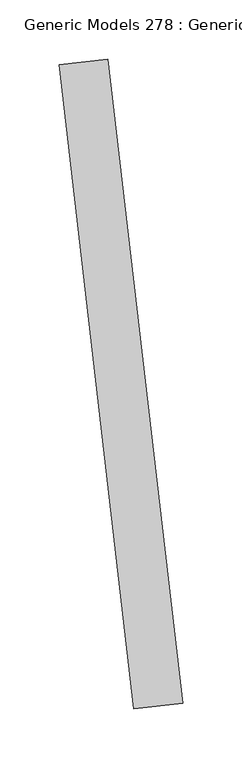
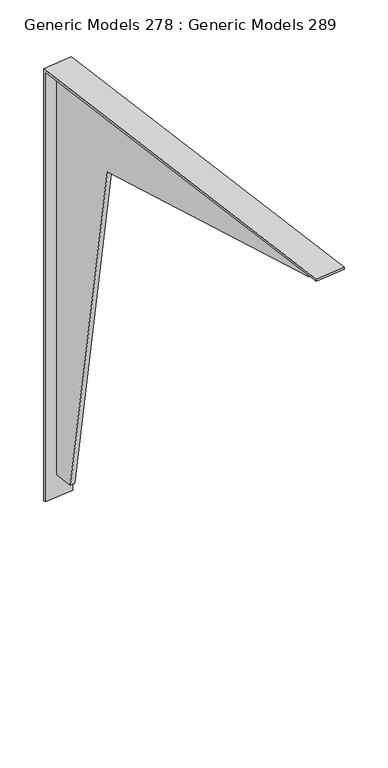
"""IFC4 building model written with IfcOpenShell, lengths in millimetres: proxy geometry, Generic Models 278 : Generic Models 289."""

from ifc_helpers import new_model, si_unit, frame, origin, place, context, project, spatial, polyline, outline, extrude, source, transform, mapped, element, save


def generic_models_278_generic_models_289_329f02fc(model_context):
    return source(origin(), model_context, "Body", "SweptSolid", [
        extrude(outline(polyline([(98.1060659, 0.0), (98.1060659, -596.4380662), (70.9315576, -596.4380662), (-3.4908021, -95.9091892), (-407.9025285, -22.6069609), (-407.9025285, 0.0), (98.1060659, 0.0)])), frame((-1150.4311232, -22429.6249942, 796.925), z_axis=(0.993316067089831, 0.11542612729009999, 0.0), x_axis=(-0.11542612729009999, 0.993316067089831, 0.0)), (0.0, 0.0, 1.0), 6.3961553),
        extrude(outline(polyline([(0.0, 0.0), (0.0, -547.7405886), (-632.0051767, -547.7405886), (-632.0051767, -544.6409847), (-3.175, -544.6409847), (-3.175, 0.0), (0.0, 0.0)])), frame((-1116.0829847, -22875.1732552, 800.1), z_axis=(0.993316067089831, 0.11542612729009999, 0.0), x_axis=(0.0, 0.0, 1.0)), (0.0, 0.0, 1.0), 41.275),
    ])


if __name__ == "__main__":
    model = new_model("IFC4")
    model_context = context("Model", 3, world=origin())
    ifc_project = project(units=[si_unit("LENGTHUNIT", "METRE", prefix="MILLI")], contexts=[model_context])
    site = spatial("IfcSite", under=ifc_project)
    building = spatial("IfcBuilding", under=site)
    placement = place(None, origin())
    generic_models_278_generic_models_289_shape = generic_models_278_generic_models_289_329f02fc(model_context)
    element("IfcBuildingElementProxy", 1, Name="Generic Models 278 : Generic Models 289", ObjectType="Generic Models 278 : Generic Models 289", at=placement, inside=building, context=model_context, shape_type="MappedRepresentation", body=[
        mapped(generic_models_278_generic_models_289_shape, transform((0.0, 0.0, 0.0), x_axis=(1.0, 0.0, 0.0), y_axis=(0.0, 1.0, 0.0), z_axis=(0.0, 0.0, 1.0))),
    ])
    save(model, "model.ifc")

# Revit data of these elements
# Element 1 (IfcBuildingElementProxy, "Generic Models 278 : Generic Models 289")
#   Materials on its faces: "ANGLE BRAKET AS NEEDED"
# Materials
#   "ANGLE BRAKET AS NEEDED": class "Metal", colour RGB 244 244 244, transparency 0, Description = "Aluminum 6061", Cost = 0
